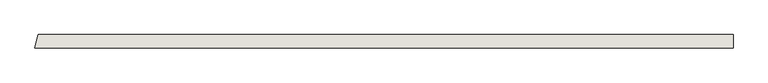
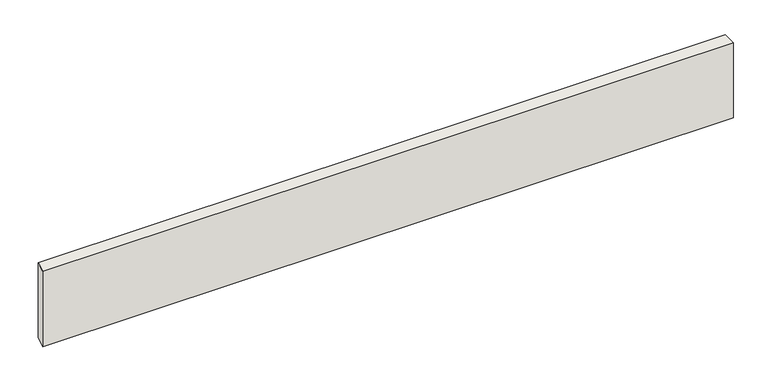
"""IFC4 building model written with IfcOpenShell, lengths in millimetres: wall geometry, Holzwand."""

import ifcopenshell
import ifcopenshell.guid

model = None  # the IFC model being written
_history = None  # IfcOwnerHistory: only IFC2X3 demands one
_inside = {}  # id of a spatial element -> (the spatial element, [elements in it])
_under = {}  # id of a project, library or spatial element -> (it, [spatial elements below it])
_declared = {}  # id of a project -> (the project, [libraries it declares])
_typed = {}  # id of a type object -> (the type object, [elements of that type])
_made_of = {}  # id of a material, layer set ... -> (it, [elements and type objects made of it])


def new_model(schema):
    """Start an empty IFC model of exactly this schema.

    Asked for "IFC4X3", IfcOpenShell would pick the latest addendum, in which some entities
    have other attributes; the version numbers below select the first issue.
    IFC2X3 requires an IfcOwnerHistory on every rooted entity: one is made here for all.
    """
    global model, _history
    if schema == "IFC4X3":
        model = ifcopenshell.file(schema_version=(4, 3, 0, 0))
    else:
        model = ifcopenshell.file(schema=schema)
    _inside.clear()
    _under.clear()
    _declared.clear()
    _typed.clear()
    _made_of.clear()
    _history = None
    if model.schema == "IFC2X3":
        org = make("IfcOrganization", Name="unknown")
        user = make(
            "IfcPersonAndOrganization",
            ThePerson=make("IfcPerson", FamilyName="unknown"),
            TheOrganization=org,
        )
        app = make(
            "IfcApplication",
            ApplicationDeveloper=org,
            Version="unknown",
            ApplicationFullName="unknown",
            ApplicationIdentifier="unknown",
        )
        _history = make(
            "IfcOwnerHistory",
            OwningUser=user,
            OwningApplication=app,
            ChangeAction="ADDED",
            CreationDate=0,
        )
    return model


def make(cls, **values):
    """One entity of the class cls with the attributes given. An attribute that is None is left unset."""
    return model.create_entity(
        cls, **{name: value for name, value in values.items() if value is not None}
    )


def rooted(cls, **values):
    """An entity with a GlobalId (a new one), such as an element, a storey or a relation."""
    return make(cls, GlobalId=ifcopenshell.guid.new(), OwnerHistory=_history, **values)


def si_unit(unit_type, name, prefix=None):
    """IfcSIUnit, for example si_unit("LENGTHUNIT", "METRE", prefix="MILLI")."""
    return make("IfcSIUnit", UnitType=unit_type, Prefix=prefix, Name=name)


def assignment(units):
    """IfcUnitAssignment: the units of a project."""
    return None if units is None else make("IfcUnitAssignment", Units=units)


def point(xyz):
    """IfcCartesianPoint."""
    return None if xyz is None else make("IfcCartesianPoint", Coordinates=xyz)


def direction(xyz):
    """IfcDirection."""
    return None if xyz is None else make("IfcDirection", DirectionRatios=xyz)


def frame(location, z_axis=None, x_axis=None):
    """IfcAxis2Placement3D, a coordinate frame: its origin and axes. An axis left out is left unset."""
    return make(
        "IfcAxis2Placement3D",
        Location=point(location),
        Axis=direction(z_axis),
        RefDirection=direction(x_axis),
    )


def origin():
    """The frame at (0, 0, 0) with its axes left unset."""
    return frame((0.0, 0.0, 0.0))


def origin_with_axes():
    """The frame at (0, 0, 0) with the z axis (0, 0, 1) and the x axis (1, 0, 0) written out."""
    return frame((0.0, 0.0, 0.0), z_axis=(0.0, 0.0, 1.0), x_axis=(1.0, 0.0, 0.0))


def place(relative_to, where):
    """IfcLocalPlacement: puts the frame where relative to a parent placement (None: the world)."""
    return make(
        "IfcLocalPlacement", PlacementRelTo=relative_to, RelativePlacement=where
    )


def context(
    kind, dimensions, precision=None, world=None, true_north=None, identifier=None
):
    """IfcGeometricRepresentationContext, for example the 3D "Model" context."""
    return make(
        "IfcGeometricRepresentationContext",
        ContextIdentifier=identifier,
        ContextType=kind,
        CoordinateSpaceDimension=dimensions,
        Precision=precision,
        WorldCoordinateSystem=world,
        TrueNorth=true_north,
    )


def project(units=None, contexts=None):
    """IfcProject with its units and contexts."""
    return rooted(
        "IfcProject",
        Name="project",
        RepresentationContexts=contexts,
        UnitsInContext=assignment(units),
    )


def spatial(cls, under=None, at=None, **own):
    """A site, building, storey or space (cls), placed at a placement, below another one or the project."""
    s = rooted(cls, ObjectPlacement=at, **own)
    if under is not None:
        _under.setdefault(under.id(), (under, []))[1].append(s)
    return s


def polyline(points):
    """IfcPolyline through the points."""
    return make("IfcPolyline", Points=[point(p) for p in points])


def outline(outer, holes=None, kind="AREA"):
    """IfcArbitraryClosedProfileDef: a profile drawn as a closed curve; with holes, ...WithVoids."""
    if holes is None:
        return make("IfcArbitraryClosedProfileDef", ProfileType=kind, OuterCurve=outer)
    return make(
        "IfcArbitraryProfileDefWithVoids",
        ProfileType=kind,
        OuterCurve=outer,
        InnerCurves=holes,
    )


def extrude(swept, where, along, depth):
    """IfcExtrudedAreaSolid: the profile swept, set in the frame where, extruded along a direction by depth."""
    return make(
        "IfcExtrudedAreaSolid",
        SweptArea=swept,
        Position=where,
        ExtrudedDirection=direction(along),
        Depth=depth,
    )


def shape(context_of_items, identifier, shape_type, items):
    """IfcShapeRepresentation: the items that make up one representation, for example the "Body"."""
    return make(
        "IfcShapeRepresentation",
        ContextOfItems=context_of_items,
        RepresentationIdentifier=identifier,
        RepresentationType=shape_type,
        Items=items,
    )


def source(mapping_origin, context_of_items, identifier, shape_type, items):
    """IfcRepresentationMap: a shape defined once, which mapped items show again and again."""
    return make(
        "IfcRepresentationMap",
        MappingOrigin=mapping_origin,
        MappedRepresentation=shape(context_of_items, identifier, shape_type, items),
    )


def transform(
    local_origin,
    x_axis=None,
    y_axis=None,
    z_axis=None,
    scale=None,
    scale2=None,
    scale3=None,
    uniform=True,
):
    """IfcCartesianTransformationOperator3D, or its non-uniform kind. x_axis, y_axis, z_axis: its Axis1, 2, 3."""
    if uniform:
        return make(
            "IfcCartesianTransformationOperator3D",
            Axis1=direction(x_axis),
            Axis2=direction(y_axis),
            LocalOrigin=point(local_origin),
            Scale=scale,
            Axis3=direction(z_axis),
        )
    return make(
        "IfcCartesianTransformationOperator3DnonUniform",
        Axis1=direction(x_axis),
        Axis2=direction(y_axis),
        LocalOrigin=point(local_origin),
        Scale=scale,
        Axis3=direction(z_axis),
        Scale2=scale2,
        Scale3=scale3,
    )


def mapped(mapping_source, mapping_target):
    """IfcMappedItem: shows the shape of a source again, moved by a transform."""
    return make(
        "IfcMappedItem", MappingSource=mapping_source, MappingTarget=mapping_target
    )


def made_of(thing, what):
    """Note that an element or type object is made of a material, layer set ...; save() writes the relation."""
    if what is not None:
        _made_of.setdefault(what.id(), (what, []))[1].append(thing)
    return thing


def element(
    cls,
    number,
    at=None,
    inside=None,
    cuts=None,
    type_object=None,
    material=None,
    context=None,
    identifier="Body",
    shape_type=None,
    held_by="IfcProductDefinitionShape",
    body=None,
    shapes=None,
    **own,
):
    """One element of the class cls, such as IfcWall. Its Tag is "e" and its number.

    at: its placement. inside: the storey or other place that contains it. cuts: it is an
    opening in that element (IfcRelVoidsElement). A single representation is given by context,
    identifier, shape_type and body (its items); several are given by shapes. held_by: the class
    of the entity that holds the representations. save() writes the other relations.
    """
    e = rooted(cls, Tag="e%d" % number, ObjectPlacement=at, **own)
    if body is not None:
        shapes = [shape(context, identifier, shape_type, body)]
    if shapes is not None:
        e.Representation = make(held_by, Representations=shapes)
    if inside is not None:
        _inside.setdefault(inside.id(), (inside, []))[1].append(e)
    if cuts is not None:
        rooted(
            "IfcRelVoidsElement", RelatingBuildingElement=cuts, RelatedOpeningElement=e
        )
    if type_object is not None:
        _typed.setdefault(type_object.id(), (type_object, []))[1].append(e)
    return made_of(e, material)


def aggregate(whole, parts):
    """IfcRelAggregates: a whole, such as a stair, and the parts it consists of."""
    return rooted("IfcRelAggregates", RelatingObject=whole, RelatedObjects=parts)


def save(model, path):
    """Write the relations noted so far, then the file.

    IfcRelAggregates (storeys below a building ...), IfcRelContainedInSpatialStructure (elements
    in a storey), IfcRelDefinesByType, IfcRelAssociatesMaterial and IfcRelDeclares: one each for
    every whole, place, type object, material and project.
    """
    for whole, parts in _under.values():
        aggregate(whole, parts)
    for where, things in _inside.values():
        rooted(
            "IfcRelContainedInSpatialStructure",
            RelatedElements=things,
            RelatingStructure=where,
        )
    for kind, things in _typed.values():
        rooted("IfcRelDefinesByType", RelatedObjects=things, RelatingType=kind)
    for what, things in _made_of.values():
        rooted("IfcRelAssociatesMaterial", RelatedObjects=things, RelatingMaterial=what)
    for by, libraries in _declared.values():
        rooted("IfcRelDeclares", RelatingContext=by, RelatedDefinitions=libraries)
    model.write(path)


def wall_7a3c9a4f(model_context):
    return source(origin(), model_context, "Body", "SweptSolid", [
        extrude(outline(polyline([(10390.1642022, 0.0), (0.0, 0.0), (48.1082675, 200.0), (10390.1642022, 200.0), (10390.1642022, 0.0)])), origin_with_axes(), (0.0, 0.0, 1.0), 1200.0),
    ])


if __name__ == "__main__":
    model = new_model("IFC4")
    model_context = context("Model", 3, world=origin())
    ifc_project = project(units=[si_unit("LENGTHUNIT", "METRE", prefix="MILLI")], contexts=[model_context])
    site = spatial("IfcSite", under=ifc_project)
    building = spatial("IfcBuilding", under=site)
    placement = place(None, origin())
    wall_shape = wall_7a3c9a4f(model_context)
    element("IfcWall", 1, ObjectType="Holzwand", at=placement, inside=building, context=model_context, shape_type="MappedRepresentation", body=[
        mapped(wall_shape, transform((0.0, 0.0, 0.0), x_axis=(1.0, 0.0, 0.0), y_axis=(0.0, 1.0, 0.0), z_axis=(0.0, 0.0, 1.0))),
    ])
    save(model, "model.ifc")

# Revit data of these elements
# Element 1 (IfcWall, "Holzwand")
#   Materials on its faces: "NC-GK-Platte-grau"
# Materials
#   "NC-GK-Platte-grau": class "Unassigned", colour RGB 199 199 199, transparency 0
